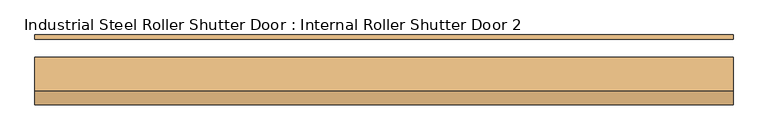
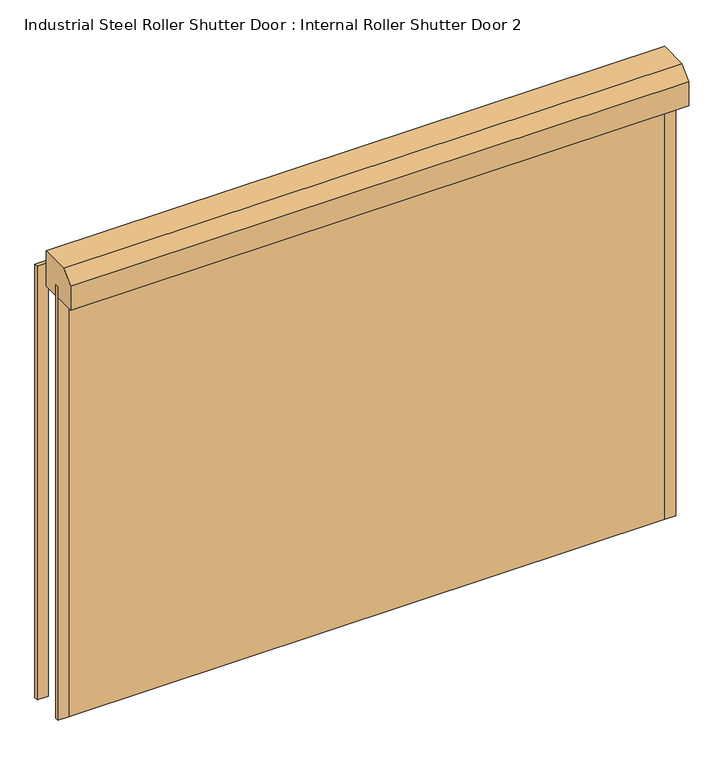
"""IFC4 building model written with IfcOpenShell, lengths in millimetres: door geometry, Industrial Steel Roller Shutter Door : Internal Roller Shutter Door 2."""

from ifc_helpers import new_model, si_unit, frame, origin, place, context, project, spatial, polyline, outline, extrude, source, transform, mapped, element, save


def industrial_steel_roller_shutter_door_internal_roller_shutter_dea29793(model_context):
    return source(origin(), model_context, "Body", "SweptSolid", [
        extrude(outline(polyline([(3000.0, -2000.0), (3000.0, 2000.0), (0.0, 2000.0), (0.0, 2075.0), (3075.0, 2075.0), (3075.0, -2075.0), (0.0, -2075.0), (0.0, -2000.0), (3000.0, -2000.0)])), frame((0.0, -132.5, 0.0), z_axis=(0.0, 1.0, 0.0), x_axis=(0.0, 0.0, 1.0)), (0.0, 0.0, 1.0), 25.0),
        extrude(outline(polyline([(3075.0, -2075.0), (0.0, -2075.0), (0.0, -2000.0), (3000.0, -2000.0), (3000.0, 2000.0), (0.0, 2000.0), (0.0, 2075.0), (3075.0, 2075.0), (3075.0, -2075.0)])), frame((0.0, 107.5, 0.0), z_axis=(0.0, 1.0, 0.0), x_axis=(0.0, 0.0, 1.0)), (0.0, 0.0, 1.0), 25.0),
        extrude(outline(polyline([(0.0, 3000.0), (0.0, 0.0), (-132.5, 0.0), (-132.5, 2975.0), (-107.5, 2975.0), (-107.5, 3000.0), (0.0, 3000.0)])), frame((-2000.0, 0.0, 0.0), z_axis=(1.0, 0.0, 0.0), x_axis=(0.0, 1.0, 0.0)), (0.0, 0.0, 1.0), 4000.0),
        extrude(outline(polyline([(0.0, 3250.0), (0.0, 3000.0), (-282.5, 3000.0), (-282.5, 3170.0), (-202.5, 3250.0), (0.0, 3250.0)])), frame((-2075.0, 0.0, 0.0), z_axis=(1.0, 0.0, 0.0), x_axis=(0.0, 1.0, 0.0)), (0.0, 0.0, 1.0), 4150.0),
    ])


if __name__ == "__main__":
    model = new_model("IFC4")
    model_context = context("Model", 3, world=origin())
    ifc_project = project(units=[si_unit("LENGTHUNIT", "METRE", prefix="MILLI")], contexts=[model_context])
    site = spatial("IfcSite", under=ifc_project)
    building = spatial("IfcBuilding", under=site)
    placement = place(None, origin())
    industrial_steel_roller_shutter_door_internal_roller_shutter_shape = industrial_steel_roller_shutter_door_internal_roller_shutter_dea29793(model_context)
    element("IfcDoor", 1, ObjectType="Industrial Steel Roller Shutter Door : Internal Roller Shutter Door 2", at=placement, inside=building, context=model_context, shape_type="MappedRepresentation", body=[
        mapped(industrial_steel_roller_shutter_door_internal_roller_shutter_shape, transform((0.0, 0.0, 0.0), x_axis=(1.0, 0.0, 0.0), y_axis=(0.0, 1.0, 0.0), z_axis=(0.0, 0.0, 1.0))),
    ])
    save(model, "model.ifc")

# Revit data of these elements
# Type "Industrial Steel Roller Shutter Door : Internal Roller Shutter Door 2"
#   Description = "Internal Roller Shutter Door"
#   Type Mark = "56"
#   Frame Projection Ext. = 25 mm
#   Frame Projection Int. = 25 mm
#   Frame Width = 75 mm
#   Height = 3000 mm
#   Width = 4000 mm
#   Function = (empty or 0)
#   Wall Closure = (empty or 0)
#   Assembly Code = ""
# Element 1 (IfcDoor, "Industrial Steel Roller Shutter Door : Internal Roller Shutter Door 2")
#   Materials on its faces: "Steel Shutters", "Render 0-255-0"
# Materials
#   "Steel Shutters": class "Vinyl", colour RGB 122 127 125, transparency 0
#   "Render 0-255-0": class "Miscellaneous", colour RGB 0 255 0, transparency 0
